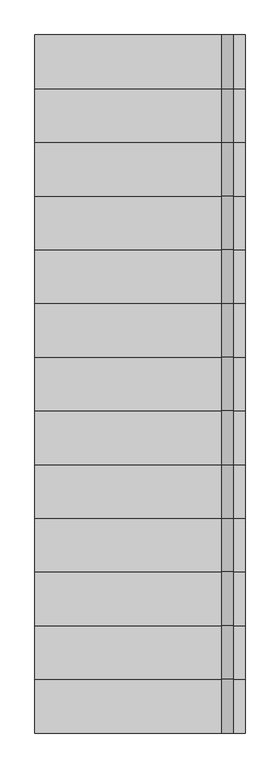
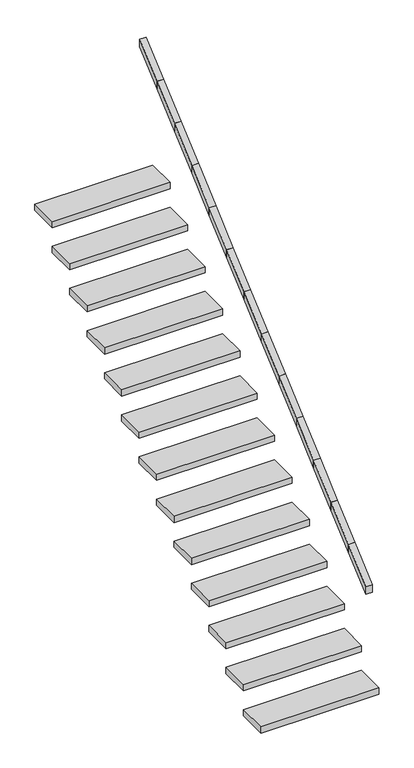
"""IFC4 building model written with IfcOpenShell, lengths in millimetres: stair geometry, 0_3d."""

from ifc_helpers import new_model, si_unit, frame, origin, origin_with_axes, place, context, project, spatial, polyline, outline, extrude, source, transform, mapped, element, save


def stair_e75a4082(model_context):
    return source(origin(), model_context, "Body", "SweptSolid", [
        extrude(outline(polyline([(1379.9989151, 2100.0), (1379.9989151, 2039.1184732), (1149.9990959, 1839.1184732), (1149.9990959, 1900.0), (1379.9989151, 2100.0)])), frame((800.0, 0.0, 0.0), z_axis=(1.0, 0.0, 0.0), x_axis=(0.0, 1.0, 0.0)), (0.0, 0.0, 1.0), 50.0),
        extrude(outline(polyline([(0.0, 2069.9983727), (0.0, 2299.9981918), (900.0, 2299.9981918), (900.0, 2069.9983727), (0.0, 2069.9983727)])), frame((0.0, 0.0, 1800.0), z_axis=(0.0, 0.0, 1.0), x_axis=(1.0, 0.0, 0.0)), (0.0, 0.0, 1.0), 50.0),
        extrude(outline(polyline([(2989.9976494, 3500.0), (2989.9976494, 3439.1184732), (2759.9978302, 3239.1184732), (2759.9978302, 3300.0), (2989.9976494, 3500.0)])), frame((800.0, 0.0, 0.0), z_axis=(1.0, 0.0, 0.0), x_axis=(0.0, 1.0, 0.0)), (0.0, 0.0, 1.0), 50.0),
        extrude(outline(polyline([(0.0, 459.9996384), (0.0, 689.9994576), (900.0, 689.9994576), (900.0, 459.9996384), (0.0, 459.9996384)])), frame((0.0, 0.0, 400.0), z_axis=(0.0, 0.0, 1.0), x_axis=(1.0, 0.0, 0.0)), (0.0, 0.0, 1.0), 50.0),
        extrude(outline(polyline([(0.0, 1379.9989151), (0.0, 1609.9987343), (900.0, 1609.9987343), (900.0, 1379.9989151), (0.0, 1379.9989151)])), frame((0.0, 0.0, 1200.0), z_axis=(0.0, 0.0, 1.0), x_axis=(1.0, 0.0, 0.0)), (0.0, 0.0, 1.0), 50.0),
        extrude(outline(polyline([(0.0, 2529.998011), (0.0, 2759.9978302), (900.0, 2759.9978302), (900.0, 2529.998011), (0.0, 2529.998011)])), frame((0.0, 0.0, 2200.0), z_axis=(0.0, 0.0, 1.0), x_axis=(1.0, 0.0, 0.0)), (0.0, 0.0, 1.0), 50.0),
        extrude(outline(polyline([(2069.9983727, 2700.0), (2069.9983727, 2639.1184732), (1839.9985535, 2439.1184732), (1839.9985535, 2500.0), (2069.9983727, 2700.0)])), frame((800.0, 0.0, 0.0), z_axis=(1.0, 0.0, 0.0), x_axis=(0.0, 1.0, 0.0)), (0.0, 0.0, 1.0), 50.0),
        extrude(outline(polyline([(2299.9981918, 2900.0), (2299.9981918, 2839.1184732), (2069.9983727, 2639.1184732), (2069.9983727, 2700.0), (2299.9981918, 2900.0)])), frame((800.0, 0.0, 0.0), z_axis=(1.0, 0.0, 0.0), x_axis=(0.0, 1.0, 0.0)), (0.0, 0.0, 1.0), 50.0),
        extrude(outline(polyline([(0.0, 1149.9990959), (0.0, 1379.9989151), (900.0, 1379.9989151), (900.0, 1149.9990959), (0.0, 1149.9990959)])), frame((0.0, 0.0, 1000.0), z_axis=(0.0, 0.0, 1.0), x_axis=(1.0, 0.0, 0.0)), (0.0, 0.0, 1.0), 50.0),
        extrude(outline(polyline([(0.0, 1609.9987343), (0.0, 1839.9985535), (900.0, 1839.9985535), (900.0, 1609.9987343), (0.0, 1609.9987343)])), frame((0.0, 0.0, 1400.0), z_axis=(0.0, 0.0, 1.0), x_axis=(1.0, 0.0, 0.0)), (0.0, 0.0, 1.0), 50.0),
        extrude(outline(polyline([(229.9998192, 1100.0), (229.9998192, 1039.1184732), (0.0, 839.1184732), (0.0, 900.0), (229.9998192, 1100.0)])), frame((800.0, 0.0, 0.0), z_axis=(1.0, 0.0, 0.0), x_axis=(0.0, 1.0, 0.0)), (0.0, 0.0, 1.0), 50.0),
        extrude(outline(polyline([(459.9996384, 1300.0), (459.9996384, 1239.1184732), (229.9998192, 1039.1184732), (229.9998192, 1100.0), (459.9996384, 1300.0)])), frame((800.0, 0.0, 0.0), z_axis=(1.0, 0.0, 0.0), x_axis=(0.0, 1.0, 0.0)), (0.0, 0.0, 1.0), 50.0),
        extrude(outline(polyline([(0.0, 2299.9981918), (0.0, 2529.998011), (900.0, 2529.998011), (900.0, 2299.9981918), (0.0, 2299.9981918)])), frame((0.0, 0.0, 2000.0), z_axis=(0.0, 0.0, 1.0), x_axis=(1.0, 0.0, 0.0)), (0.0, 0.0, 1.0), 50.0),
        extrude(outline(polyline([(0.0, 919.9992767), (0.0, 1149.9990959), (900.0, 1149.9990959), (900.0, 919.9992767), (0.0, 919.9992767)])), frame((0.0, 0.0, 800.0), z_axis=(0.0, 0.0, 1.0), x_axis=(1.0, 0.0, 0.0)), (0.0, 0.0, 1.0), 50.0),
        extrude(outline(polyline([(0.0, 689.9994576), (0.0, 919.9992767), (900.0, 919.9992767), (900.0, 689.9994576), (0.0, 689.9994576)])), frame((0.0, 0.0, 600.0), z_axis=(0.0, 0.0, 1.0), x_axis=(1.0, 0.0, 0.0)), (0.0, 0.0, 1.0), 50.0),
        extrude(outline(polyline([(2759.9978302, 3300.0), (2759.9978302, 3239.1184732), (2529.998011, 3039.1184732), (2529.998011, 3100.0), (2759.9978302, 3300.0)])), frame((800.0, 0.0, 0.0), z_axis=(1.0, 0.0, 0.0), x_axis=(0.0, 1.0, 0.0)), (0.0, 0.0, 1.0), 50.0),
        extrude(outline(polyline([(0.0, 0.0), (0.0, 229.9998192), (900.0, 229.9998192), (900.0, 0.0), (0.0, 0.0)])), origin_with_axes(), (0.0, 0.0, 1.0), 50.0),
        extrude(outline(polyline([(0.0, 1839.9985535), (0.0, 2069.9983727), (900.0, 2069.9983727), (900.0, 1839.9985535), (0.0, 1839.9985535)])), frame((0.0, 0.0, 1600.0), z_axis=(0.0, 0.0, 1.0), x_axis=(1.0, 0.0, 0.0)), (0.0, 0.0, 1.0), 50.0),
        extrude(outline(polyline([(0.0, 229.9998192), (0.0, 459.9996384), (900.0, 459.9996384), (900.0, 229.9998192), (0.0, 229.9998192)])), frame((0.0, 0.0, 200.0), z_axis=(0.0, 0.0, 1.0), x_axis=(1.0, 0.0, 0.0)), (0.0, 0.0, 1.0), 50.0),
        extrude(outline(polyline([(0.0, 2759.9978302), (0.0, 2989.9976494), (900.0, 2989.9976494), (900.0, 2759.9978302), (0.0, 2759.9978302)])), frame((0.0, 0.0, 2400.0), z_axis=(0.0, 0.0, 1.0), x_axis=(1.0, 0.0, 0.0)), (0.0, 0.0, 1.0), 50.0),
        extrude(outline(polyline([(2529.998011, 3100.0), (2529.998011, 3039.1184732), (2299.9981918, 2839.1184732), (2299.9981918, 2900.0), (2529.998011, 3100.0)])), frame((800.0, 0.0, 0.0), z_axis=(1.0, 0.0, 0.0), x_axis=(0.0, 1.0, 0.0)), (0.0, 0.0, 1.0), 50.0),
        extrude(outline(polyline([(1609.9987343, 2300.0), (1609.9987343, 2239.1184732), (1379.9989151, 2039.1184732), (1379.9989151, 2100.0), (1609.9987343, 2300.0)])), frame((800.0, 0.0, 0.0), z_axis=(1.0, 0.0, 0.0), x_axis=(0.0, 1.0, 0.0)), (0.0, 0.0, 1.0), 50.0),
        extrude(outline(polyline([(689.9994576, 1500.0), (689.9994576, 1439.1184732), (459.9996384, 1239.1184732), (459.9996384, 1300.0), (689.9994576, 1500.0)])), frame((800.0, 0.0, 0.0), z_axis=(1.0, 0.0, 0.0), x_axis=(0.0, 1.0, 0.0)), (0.0, 0.0, 1.0), 50.0),
        extrude(outline(polyline([(1839.9985535, 2500.0), (1839.9985535, 2439.1184732), (1609.9987343, 2239.1184732), (1609.9987343, 2300.0), (1839.9985535, 2500.0)])), frame((800.0, 0.0, 0.0), z_axis=(1.0, 0.0, 0.0), x_axis=(0.0, 1.0, 0.0)), (0.0, 0.0, 1.0), 50.0),
        extrude(outline(polyline([(1149.9990959, 1900.0), (1149.9990959, 1839.1184732), (919.9992767, 1639.1184732), (919.9992767, 1700.0), (1149.9990959, 1900.0)])), frame((800.0, 0.0, 0.0), z_axis=(1.0, 0.0, 0.0), x_axis=(0.0, 1.0, 0.0)), (0.0, 0.0, 1.0), 50.0),
        extrude(outline(polyline([(919.9992767, 1700.0), (919.9992767, 1639.1184732), (689.9994576, 1439.1184732), (689.9994576, 1500.0), (919.9992767, 1700.0)])), frame((800.0, 0.0, 0.0), z_axis=(1.0, 0.0, 0.0), x_axis=(0.0, 1.0, 0.0)), (0.0, 0.0, 1.0), 50.0),
    ])


if __name__ == "__main__":
    model = new_model("IFC4")
    model_context = context("Model", 3, world=origin())
    ifc_project = project(units=[si_unit("LENGTHUNIT", "METRE", prefix="MILLI")], contexts=[model_context])
    site = spatial("IfcSite", under=ifc_project)
    building = spatial("IfcBuilding", under=site)
    placement = place(None, origin())
    stair_shape = stair_e75a4082(model_context)
    element("IfcStair", 1, ObjectType="0_3d", at=placement, inside=building, context=model_context, shape_type="MappedRepresentation", body=[
        mapped(stair_shape, transform((0.0, 0.0, 0.0), x_axis=(1.0, 0.0, 0.0), y_axis=(0.0, 1.0, 0.0), z_axis=(0.0, 0.0, 1.0))),
    ])
    save(model, "model.ifc")

# Revit data of these elements
# Element 1 (IfcStair, "0_3d")
#   Materials on its faces: "*1", "weiss"
# Materials
#   "*1": class "Unassigned", colour RGB 175 175 175, transparency 0
#   "weiss": class "Unassigned", colour RGB 255 255 255, transparency 0
